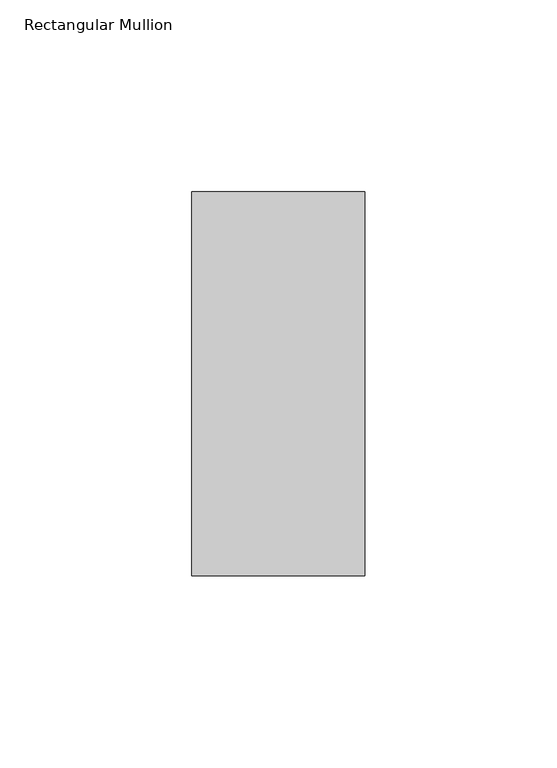
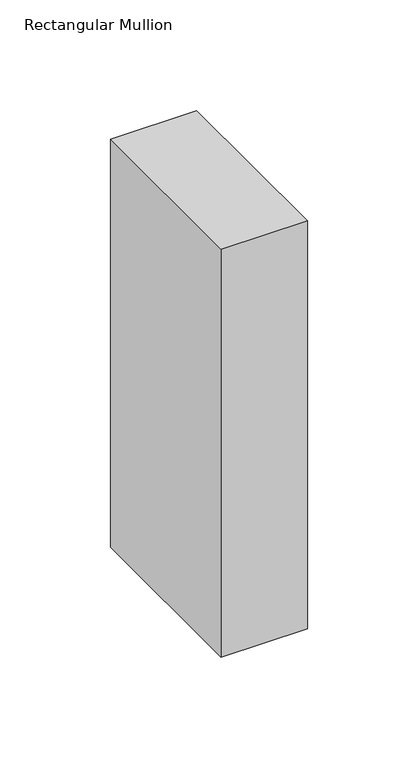
"""IFC4 building model written with IfcOpenShell, lengths in millimetres: member geometry, Rectangular Mullion : 알루미늄_Rectangular Cap_100 x 45."""

from ifc_helpers import new_model, si_unit, frame, origin, place, context, project, spatial, polyline, outline, extrude, source, transform, mapped, element, save


def rectangular_mullion_4e3af655(model_context):
    return source(origin(), model_context, "Body", "SweptSolid", [
        extrude(outline(polyline([(0.0, 50.0), (0.0, -50.0), (-45.0, -50.0), (-45.0, 50.0), (0.0, 50.0)])), frame((0.0, 0.0, -225.0000001), z_axis=(0.0, 0.0, 1.0), x_axis=(1.0, 0.0, 0.0)), (0.0, 0.0, 1.0), 225.0000001),
    ])


if __name__ == "__main__":
    model = new_model("IFC4")
    model_context = context("Model", 3, world=origin())
    ifc_project = project(units=[si_unit("LENGTHUNIT", "METRE", prefix="MILLI")], contexts=[model_context])
    site = spatial("IfcSite", under=ifc_project)
    building = spatial("IfcBuilding", under=site)
    placement = place(None, origin())
    rectangular_mullion_shape = rectangular_mullion_4e3af655(model_context)
    element("IfcMember", 1, ObjectType="Rectangular Mullion : 알루미늄_Rectangular Cap_100 x 45", at=placement, inside=building, context=model_context, shape_type="MappedRepresentation", body=[
        mapped(rectangular_mullion_shape, transform((0.0, 0.0, 0.0), x_axis=(1.0, 0.0, 0.0), y_axis=(0.0, 1.0, 0.0), z_axis=(0.0, 0.0, 1.0))),
    ])
    save(model, "model.ifc")

# Revit data of these elements
# Type "Rectangular Mullion : 알루미늄_Rectangular Cap_100 x 45"
#   built-in parameter 1007304 = 0.328084 (stored number, unit not read)
#   built-in parameter 1007301 = 0.0738189 (stored number, unit not read)
#   built-in parameter 1007300 = 0.0738189 (stored number, unit not read)
# Element 1 (IfcMember, "Rectangular Mullion : 알루미늄_Rectangular Cap_100 x 45")
#   Materials on its faces: "00_Metal_Stainless Steel"
# Materials
#   "00_Metal_Stainless Steel": class "Metal", colour RGB 148 148 148, transparency 0, Description = "Steel", Cost = 0
